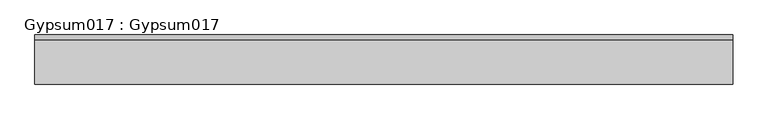
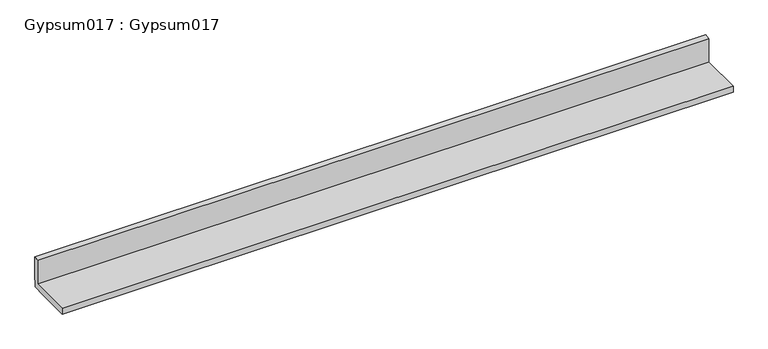
"""IFC4 building model written with IfcOpenShell, lengths in millimetres: proxy geometry, Gypsum017 : Gypsum017."""

from ifc_helpers import new_model, si_unit, frame, origin, place, context, project, spatial, polyline, outline, extrude, source, transform, mapped, element, save


def gypsum017_gypsum017_1a790526(model_context):
    return source(origin(), model_context, "Body", "SweptSolid", [
        extrude(outline(polyline([(-4376.7836914, 42583.1921875), (-4376.7836914, 42601.896), (-4250.2279008, 42601.896), (-4250.2279008, 42675.5351562), (-4235.9495263, 42678.9921875), (-4235.9495263, 42605.6253714), (-4237.2648904, 42605.6253714), (-4237.2648904, 42584.4721875), (-4258.4180743, 42584.4721875), (-4258.4180743, 42583.1921875), (-4376.7836914, 42583.1921875)])), frame((12383.0178845, 0.0, 0.0), z_axis=(1.0, 0.0, 0.0), x_axis=(0.0, 1.0, 0.0)), (0.0, 0.0, 1.0), 2000.0),
    ])


if __name__ == "__main__":
    model = new_model("IFC4")
    model_context = context("Model", 3, world=origin())
    ifc_project = project(units=[si_unit("LENGTHUNIT", "METRE", prefix="MILLI")], contexts=[model_context])
    site = spatial("IfcSite", under=ifc_project)
    building = spatial("IfcBuilding", under=site)
    placement = place(None, origin())
    gypsum017_gypsum017_shape = gypsum017_gypsum017_1a790526(model_context)
    element("IfcBuildingElementProxy", 1, Name="Gypsum017 : Gypsum017", ObjectType="Gypsum017 : Gypsum017", at=placement, inside=building, context=model_context, shape_type="MappedRepresentation", body=[
        mapped(gypsum017_gypsum017_shape, transform((0.0, 0.0, 0.0), x_axis=(1.0, 0.0, 0.0), y_axis=(0.0, 1.0, 0.0), z_axis=(0.0, 0.0, 1.0))),
    ])
    save(model, "model.ifc")

# Revit data of these elements
# Type "Gypsum017 : Gypsum017"
#   NameOverride = "Gypsum017"
# Element 1 (IfcBuildingElementProxy, "Gypsum017 : Gypsum017")
#   Materials on its faces: "5/8\"  GYPSUM BOARD"
# Materials
#   "5/8\"  GYPSUM BOARD": class "Unassigned", colour RGB 255 255 255, transparency 0, Cost = 0
